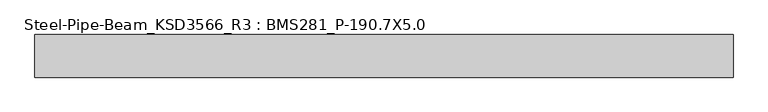
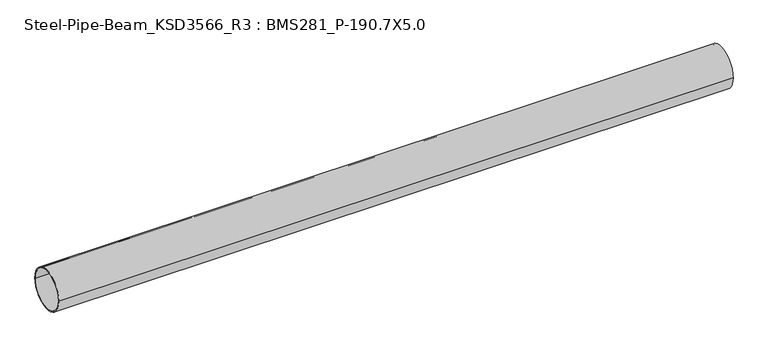
"""IFC4 building model written with IfcOpenShell, lengths in millimetres: member geometry, Steel-Pipe-Beam_KSD3566_R3 : BMS281_P-190.7X5.0."""

from ifc_helpers import new_model, si_unit, point, frame, origin, origin_2d, place, context, project, spatial, circle_curve, trimmed, segment, composite_curve, outline, extrude, source, transform, mapped, element, save


def steel_pipe_beam_ksd3566_r3_bms281_p_190_7x5_0_3761cd2c(model_context):
    return source(origin(), model_context, "Body", "SweptSolid", [
        extrude(outline(composite_curve([segment(trimmed(circle_curve(origin_2d(), 95.35), [point((-95.35, 0.0))], [point((95.35, 0.0))], False, "CARTESIAN"), True, "CONTINUOUS"), segment(trimmed(circle_curve(origin_2d(), 95.35), [point((95.35, 0.0))], [point((-95.35, 0.0))], False, "CARTESIAN"), True, "CONTINUOUS")], self_intersect=False), holes=[composite_curve([segment(trimmed(circle_curve(origin_2d(), 90.35), [point((90.35, 0.0))], [point((-90.35, 0.0))], True, "CARTESIAN"), True, "CONTINUOUS"), segment(trimmed(circle_curve(origin_2d(), 90.35), [point((-90.35, 0.0))], [point((90.35, 0.0))], True, "CARTESIAN"), True, "CONTINUOUS")], self_intersect=False)]), frame((-1487.6758865, 0.0, 0.0), z_axis=(1.0, 0.0, 0.0), x_axis=(0.0, 1.0, 0.0)), (0.0, 0.0, 1.0), 3121.8221627),
    ])


if __name__ == "__main__":
    model = new_model("IFC4")
    model_context = context("Model", 3, world=origin())
    ifc_project = project(units=[si_unit("LENGTHUNIT", "METRE", prefix="MILLI")], contexts=[model_context])
    site = spatial("IfcSite", under=ifc_project)
    building = spatial("IfcBuilding", under=site)
    placement = place(None, origin())
    steel_pipe_beam_ksd3566_r3_bms281_p_190_7x5_0_shape = steel_pipe_beam_ksd3566_r3_bms281_p_190_7x5_0_3761cd2c(model_context)
    element("IfcMember", 1, ObjectType="Steel-Pipe-Beam_KSD3566_R3 : BMS281_P-190.7X5.0", at=placement, inside=building, context=model_context, shape_type="MappedRepresentation", body=[
        mapped(steel_pipe_beam_ksd3566_r3_bms281_p_190_7x5_0_shape, transform((0.0, 0.0, 0.0), x_axis=(1.0, 0.0, 0.0), y_axis=(0.0, 1.0, 0.0), z_axis=(0.0, 0.0, 1.0))),
    ])
    save(model, "model.ifc")

# Revit data of these elements
# Type "Steel-Pipe-Beam_KSD3566_R3 : BMS281_P-190.7X5.0"
#   Keynote = "P-190.7X5.0"
#   SteelWeight = "Light"
#   t = 0.0050 m
#   Surface Area = 0.599102 m²/m
#   Section Area = 29.1697 cm²
#   Mass per Unit Length = 22.8982 kg/m
#   Length [instance default] = 1.5000 m
#   D = 0.1907 m
#   hec_material4 [instance default] = none
#   hec_material3 [instance default] = none
#   hec_material2 [instance default] = none
#   hec_material1 [instance default] = none
#   Structural Material [instance default] = Steel, 45-345
#   Assembly Code = ""
# Element 1 (IfcMember, "Steel-Pipe-Beam_KSD3566_R3 : BMS281_P-190.7X5.0")
#   Structural Material = none
# Materials
#   "Steel, 45-345": class "Metal", colour RGB 189 187 185, transparency 0, Description = "Steel 345 MPa", Cost = 0
